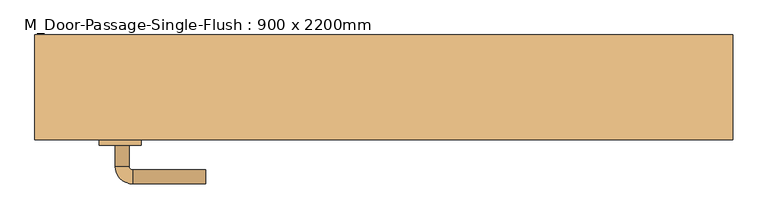
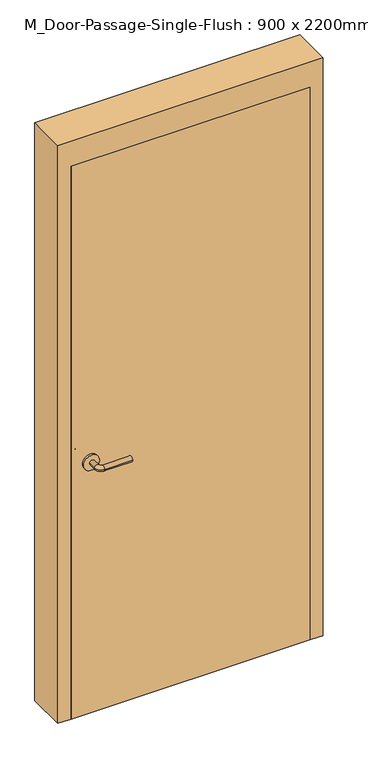
"""IFC4 building model written with IfcOpenShell, lengths in millimetres: door geometry, M_Door-Passage-Single-Flush : 900 x 2200mm."""

from ifc_helpers import new_model, si_unit, point, frame, frame_2d, origin, origin_with_axes, place, context, project, spatial, polyline, circle_curve, ellipse_curve, trimmed, segment, composite_curve, outline, extrude, faceted_brep, source, transform, mapped, element, save
from ifc_brep_helpers import plane_surface, cylinder_surface, revolved_surface, advanced_brep


def m_door_passage_single_flush_900_x_2200mm_d0d6611c(model_context):
    return source(origin(), model_context, "Body", "SolidModel", [
        advanced_brep(
        [(-384.990625, -28.35, 1000.0), (-364.990625, -28.35, 1000.0), (-384.990625, 1.65, 1000.0), (-364.990625, 1.65, 1000.0), (-359.990625, 6.65, 1000.0), (-359.990625, 26.65, 1000.0), (-254.990625, 26.65, 1000.0), (-254.990625, 6.65, 1000.0)],
        [
            (0, 1, circle_curve(frame((-374.990625, -28.35, 1000.0), z_axis=(0.0, -1.0, 0.0), x_axis=(1.0, 0.0, 0.0)), 10.0)),
            (1, 0, circle_curve(frame((-374.990625, -28.35, 1000.0), z_axis=(0.0, -1.0, 0.0), x_axis=(1.0, 0.0, 0.0)), 10.0)),
            (0, 2),
            (2, 3, circle_curve(frame((-374.990625, 1.65, 1000.0), z_axis=(0.0, -1.0, 0.0), x_axis=(1.0, 0.0, 0.0)), 10.0)),
            (3, 1),
            (3, 2, circle_curve(frame((-374.990625, 1.65, 1000.0), z_axis=(0.0, -1.0, 0.0), x_axis=(1.0, 0.0, 0.0)), 10.0)),
            (4, 3, circle_curve(frame((-359.990625, 1.65, 1000.0), z_axis=(0.0, 0.0, 1.0), x_axis=(-1.0, 0.0, 0.0)), 5.0)),
            (2, 5, circle_curve(frame((-359.990625, 1.65, 1000.0), z_axis=(0.0, 0.0, -1.0), x_axis=(-1.0, 0.0, 0.0)), 25.0)),
            (5, 4, circle_curve(frame((-359.990625, 16.65, 1000.0), z_axis=(-1.0, 0.0, 0.0), x_axis=(0.0, -1.0, 0.0)), 10.0)),
            (4, 5, circle_curve(frame((-359.990625, 16.65, 1000.0), z_axis=(-1.0, 0.0, 0.0), x_axis=(0.0, -1.0, 0.0)), 10.0)),
            (6, 7, circle_curve(frame((-254.990625, 16.65, 1000.0), z_axis=(1.0, 0.0, 0.0), x_axis=(0.0, -1.0, 0.0)), 10.0)),
            (7, 6, circle_curve(frame((-254.990625, 16.65, 1000.0), z_axis=(1.0, 0.0, 0.0), x_axis=(0.0, -1.0, 0.0)), 10.0)),
            (5, 6),
            (7, 4),
        ],
        [
            plane_surface(frame((-374.990625, -28.35, 1000.0), z_axis=(0.0, -1.0, 0.0), x_axis=(0.0, 0.0, 1.0))),
            cylinder_surface(frame((-374.990625, -28.35, 1000.0), z_axis=(0.0, -1.0, 0.0), x_axis=(1.0, 0.0, 0.0)), 10.0),
            revolved_surface(trimmed(ellipse_curve(frame((-374.990625, 1.65, 1000.0), z_axis=(0.0, -1.0, 0.0), x_axis=(1.0, 0.0, 0.0)), 10.0, 10.0), [point((-384.990625, 1.65, 1000.0))], [point((-364.990625, 1.65, 1000.0))], True, "CARTESIAN"), (-359.990625, 1.65, 1000.0), (0.0, 0.0, -1.0)),
            revolved_surface(trimmed(ellipse_curve(frame((-374.990625, 1.65, 1000.0), z_axis=(0.0, -1.0, 0.0), x_axis=(1.0, 0.0, 0.0)), 10.0, 10.0), [point((-364.990625, 1.65, 1000.0))], [point((-384.990625, 1.65, 1000.0))], True, "CARTESIAN"), (-359.990625, 1.65, 1000.0), (0.0, 0.0, -1.0)),
            plane_surface(frame((-254.990625, 16.65, 1000.0), z_axis=(1.0, 0.0, 0.0), x_axis=(0.0, 0.0, 1.0))),
            cylinder_surface(frame((-359.990625, 16.65, 1000.0), z_axis=(-1.0, 0.0, 0.0), x_axis=(0.0, -1.0, 0.0)), 10.0),
        ],
        [
            (0, [[1, 2]]),
            (1, [[-1, 3, 4, 5]]),
            (1, [[-2, -5, 6, -3]]),
            (2, [[7, -4, 8, 9]]),
            (3, [[-8, -6, -7, 10]]),
            (4, [[11, 12]]),
            (5, [[-9, 13, -12, 14]]),
            (5, [[-10, -14, -11, -13]]),
        ],
    ),
        extrude(outline(composite_curve([segment(trimmed(circle_curve(frame_2d((1000.0, -377.490625)), 30.0), [point((1000.0, -407.490625))], [point((1000.0, -347.490625))], False, "CARTESIAN"), True, "CONTINUOUS"), segment(trimmed(circle_curve(frame_2d((1000.0, -377.490625)), 30.0), [point((1000.0, -347.490625))], [point((1000.0, -407.490625))], False, "CARTESIAN"), True, "CONTINUOUS")], self_intersect=False)), frame((0.0, -36.35, 0.0), z_axis=(0.0, 1.0, 0.0), x_axis=(0.0, 0.0, 1.0)), (0.0, 0.0, 1.0), 8.0),
        advanced_brep(
        [(-384.990625, -89.35, 1000.0), (-364.990625, -89.35, 1000.0), (-364.990625, -119.35, 1000.0), (-384.990625, -119.35, 1000.0), (-359.990625, -124.35, 1000.0), (-359.990625, -144.35, 1000.0), (-254.990625, -144.35, 1000.0), (-254.990625, -124.35, 1000.0)],
        [
            (0, 1, circle_curve(frame((-374.990625, -89.35, 1000.0), z_axis=(0.0, 1.0, 0.0), x_axis=(1.0, 0.0, 0.0)), 10.0)),
            (1, 0, circle_curve(frame((-374.990625, -89.35, 1000.0), z_axis=(0.0, 1.0, 0.0), x_axis=(1.0, 0.0, 0.0)), 10.0)),
            (1, 2),
            (2, 3, circle_curve(frame((-374.990625, -119.35, 1000.0), z_axis=(0.0, 1.0, 0.0), x_axis=(1.0, 0.0, 0.0)), 10.0)),
            (3, 0),
            (3, 2, circle_curve(frame((-374.990625, -119.35, 1000.0), z_axis=(0.0, 1.0, 0.0), x_axis=(1.0, 0.0, 0.0)), 10.0)),
            (4, 5, circle_curve(frame((-359.990625, -134.35, 1000.0), z_axis=(-1.0, 0.0, 0.0), x_axis=(0.0, 1.0, 0.0)), 10.0)),
            (5, 3, circle_curve(frame((-359.990625, -119.35, 1000.0), z_axis=(0.0, 0.0, -1.0), x_axis=(-1.0, 0.0, 0.0)), 25.0)),
            (2, 4, circle_curve(frame((-359.990625, -119.35, 1000.0), z_axis=(0.0, 0.0, 1.0), x_axis=(-1.0, 0.0, 0.0)), 5.0)),
            (5, 4, circle_curve(frame((-359.990625, -134.35, 1000.0), z_axis=(-1.0, 0.0, 0.0), x_axis=(0.0, 1.0, 0.0)), 10.0)),
            (6, 7, circle_curve(frame((-254.990625, -134.35, 1000.0), z_axis=(1.0, 0.0, 0.0), x_axis=(0.0, 1.0, 0.0)), 10.0)),
            (7, 6, circle_curve(frame((-254.990625, -134.35, 1000.0), z_axis=(1.0, 0.0, 0.0), x_axis=(0.0, 1.0, 0.0)), 10.0)),
            (4, 7),
            (6, 5),
        ],
        [
            plane_surface(frame((-374.990625, -89.35, 1000.0), z_axis=(0.0, 1.0, 0.0), x_axis=(0.0, 0.0, 1.0))),
            cylinder_surface(frame((-374.990625, -89.35, 1000.0), z_axis=(0.0, 1.0, 0.0), x_axis=(1.0, 0.0, 0.0)), 10.0),
            revolved_surface(trimmed(ellipse_curve(frame((-374.990625, -119.35, 1000.0), z_axis=(0.0, -1.0, 0.0), x_axis=(1.0, 0.0, 0.0)), 10.0, 10.0), [point((-384.990625, -119.35, 1000.0))], [point((-364.990625, -119.35, 1000.0))], True, "CARTESIAN"), (-359.990625, -119.35, 1000.0), (0.0, 0.0, -1.0)),
            revolved_surface(trimmed(ellipse_curve(frame((-374.990625, -119.35, 1000.0), z_axis=(0.0, -1.0, 0.0), x_axis=(1.0, 0.0, 0.0)), 10.0, 10.0), [point((-364.990625, -119.35, 1000.0))], [point((-384.990625, -119.35, 1000.0))], True, "CARTESIAN"), (-359.990625, -119.35, 1000.0), (0.0, 0.0, -1.0)),
            plane_surface(frame((-254.990625, -134.35, 1000.0), z_axis=(1.0, 0.0, 0.0), x_axis=(0.0, 0.0, 1.0))),
            cylinder_surface(frame((-359.990625, -134.35, 1000.0), z_axis=(-1.0, 0.0, 0.0), x_axis=(0.0, 1.0, 0.0)), 10.0),
        ],
        [
            (0, [[1, 2]]),
            (1, [[3, 4, 5, -2]]),
            (1, [[-5, 6, -3, -1]]),
            (2, [[7, 8, -4, 9]]),
            (3, [[10, -9, -6, -8]]),
            (4, [[11, 12]]),
            (5, [[13, -11, 14, -7]]),
            (5, [[-14, -12, -13, -10]]),
        ],
    ),
        extrude(outline(composite_curve([segment(trimmed(circle_curve(frame_2d((1000.0, -377.490625)), 30.0), [point((1000.0, -407.490625))], [point((1000.0, -347.490625))], False, "CARTESIAN"), True, "CONTINUOUS"), segment(trimmed(circle_curve(frame_2d((1000.0, -377.490625)), 30.0), [point((1000.0, -347.490625))], [point((1000.0, -407.490625))], False, "CARTESIAN"), True, "CONTINUOUS")], self_intersect=False)), frame((0.0, -89.35, 0.0), z_axis=(0.0, 1.0, 0.0), x_axis=(0.0, 0.0, 1.0)), (0.0, 0.0, 1.0), 8.0),
        extrude(outline(polyline([(450.0, -36.35), (450.0, -81.35), (-450.0, -81.35), (-450.0, -36.35), (450.0, -36.35)])), origin_with_axes(), (0.0, 0.0, 1.0), 2200.0),
        faceted_brep([(450.0, -31.5875, 0.0), (434.125, -31.5875, 0.0), (434.125, 19.4375, 0.0), (450.0, 19.4375, 0.0), (450.0, 68.65, 0.0), (500.0, 68.65, 0.0), (500.0, -81.35, 0.0), (450.0, -81.35, 0.0), (450.0, -81.35, 2200.0), (450.0, -31.5875, 2200.0), (500.0, -81.35, 2300.0), (-500.0, -81.35, 2300.0), (-500.0, -81.35, 0.0), (-450.0, -81.35, 0.0), (-450.0, -81.35, 2200.0), (500.0, 68.65, 2300.0), (450.0, 68.65, 2200.0), (-450.0, 68.65, 2200.0), (-450.0, 68.65, 0.0), (-500.0, 68.65, 0.0), (-500.0, 68.65, 2300.0), (450.0, 19.4375, 2200.0), (434.125, 19.4375, 2184.125), (-434.125, 19.4375, 2184.125), (-434.125, 19.4375, 0.0), (-450.0, 19.4375, 0.0), (-450.0, 19.4375, 2200.0), (434.125, -31.5875, 2184.125), (-450.0, -31.5875, 2200.0), (-450.0, -31.5875, 0.0), (-434.125, -31.5875, 0.0), (-434.125, -31.5875, 2184.125)], [[[0, 1, 2, 3, 4, 5, 6, 7]], [[7, 8, 9, 0]], [[6, 10, 11, 12, 13, 14, 8, 7]], [[5, 15, 10, 6]], [[4, 16, 17, 18, 19, 20, 15, 5]], [[3, 21, 16, 4]], [[2, 22, 23, 24, 25, 26, 21, 3]], [[1, 27, 22, 2]], [[0, 9, 28, 29, 30, 31, 27, 1]], [[8, 14, 28, 9]], [[16, 21, 26, 17]], [[22, 27, 31, 23]], [[12, 19, 18, 25, 24, 30, 29, 13]], [[13, 29, 28, 14]], [[11, 20, 19, 12]], [[17, 26, 25, 18]], [[23, 31, 30, 24]], [[15, 20, 11, 10]]]),
    ])


if __name__ == "__main__":
    model = new_model("IFC4")
    model_context = context("Model", 3, world=origin())
    ifc_project = project(units=[si_unit("LENGTHUNIT", "METRE", prefix="MILLI")], contexts=[model_context])
    site = spatial("IfcSite", under=ifc_project)
    building = spatial("IfcBuilding", under=site)
    placement = place(None, origin())
    m_door_passage_single_flush_900_x_2200mm_shape = m_door_passage_single_flush_900_x_2200mm_d0d6611c(model_context)
    element("IfcDoor", 1, ObjectType="M_Door-Passage-Single-Flush : 900 x 2200mm", at=placement, inside=building, context=model_context, shape_type="MappedRepresentation", body=[
        mapped(m_door_passage_single_flush_900_x_2200mm_shape, transform((0.0, 0.0, 0.0), x_axis=(1.0, 0.0, 0.0), y_axis=(0.0, 1.0, 0.0), z_axis=(0.0, 0.0, 1.0))),
    ])
    save(model, "model.ifc")

# Revit data of these elements
# Type "M_Door-Passage-Single-Flush : 900 x 2200mm"
#   Type Mark = "39"
#   Analytic Construction = "Wooden"
#   Thickness = 45 mm
#   Thermal Resistance (R) = 0.455703 (m²·K)/W
#   Swing Angle [instance default] = 90.00°
#   Strike Height = 1000 mm
#   Rough Width [instance default] = 1000 mm
#   Rough Height [instance default] = 2300 mm
#   MF Opening Height [instance default] = 100 mm
#   MF Opening Width [instance default] = 100 mm
#   Inset Calculate [instance default] = 105 mm
#   Masonry Inset [instance default] = 25 mm
#   Height = 2200 mm
#   Width = 900 mm
#   Heat Transfer Coefficient (U) = 2.19465 W/(m²·K)
#   Masonry Frame Depth = 150 mm
#   Masonry Frame [instance default] = yes
#   Function = 1
#   Dry Wall Frame [instance default] = no
#   Panel Material = Wood - Birch
#   Frame Material = Metal - Paint Finish - Grey
#   Door Handle Material = Aluminum
#   Visual Light Transmittance = 0
#   Solar Heat Gain Coefficient = 0
#   Wall Closure = (empty or 0)
# Element 1 (IfcDoor, "M_Door-Passage-Single-Flush : 900 x 2200mm")
#   Materials on its faces: "Aluminum", "Metal - Paint Finish - Grey", "Wood - Birch"
# Materials
#   "Wood - Birch": class "Wood", colour RGB 173 132 96, transparency 0, Cost = 0
#   "Metal - Paint Finish - Grey": class "Paint", colour RGB 178 178 178, transparency 0, Cost = 0
#   "Aluminum": class "Metal", colour RGB 244 245 246, transparency 0, Description = "Aluminum 6061", Cost = 0
